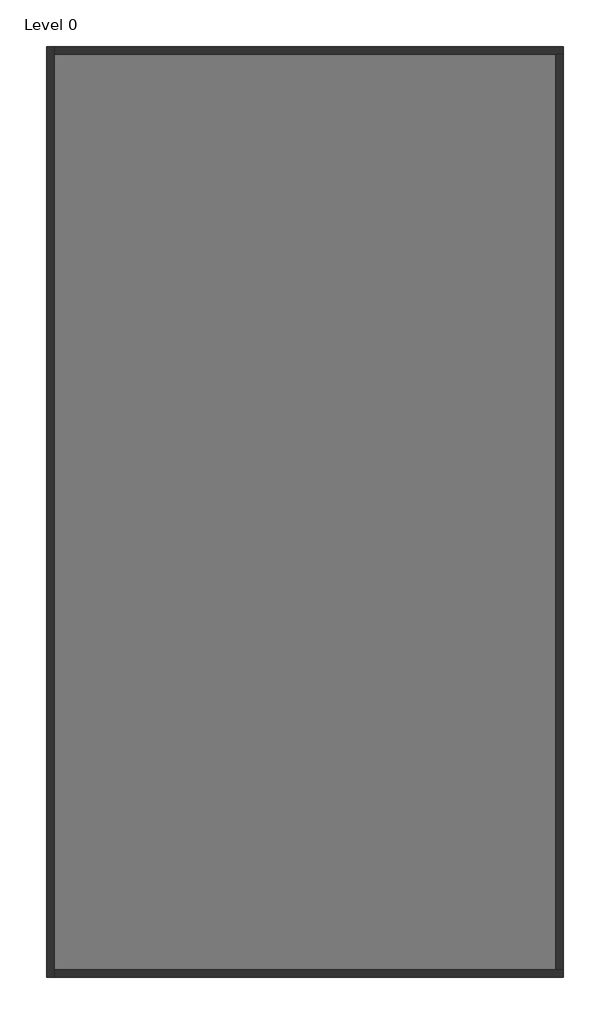
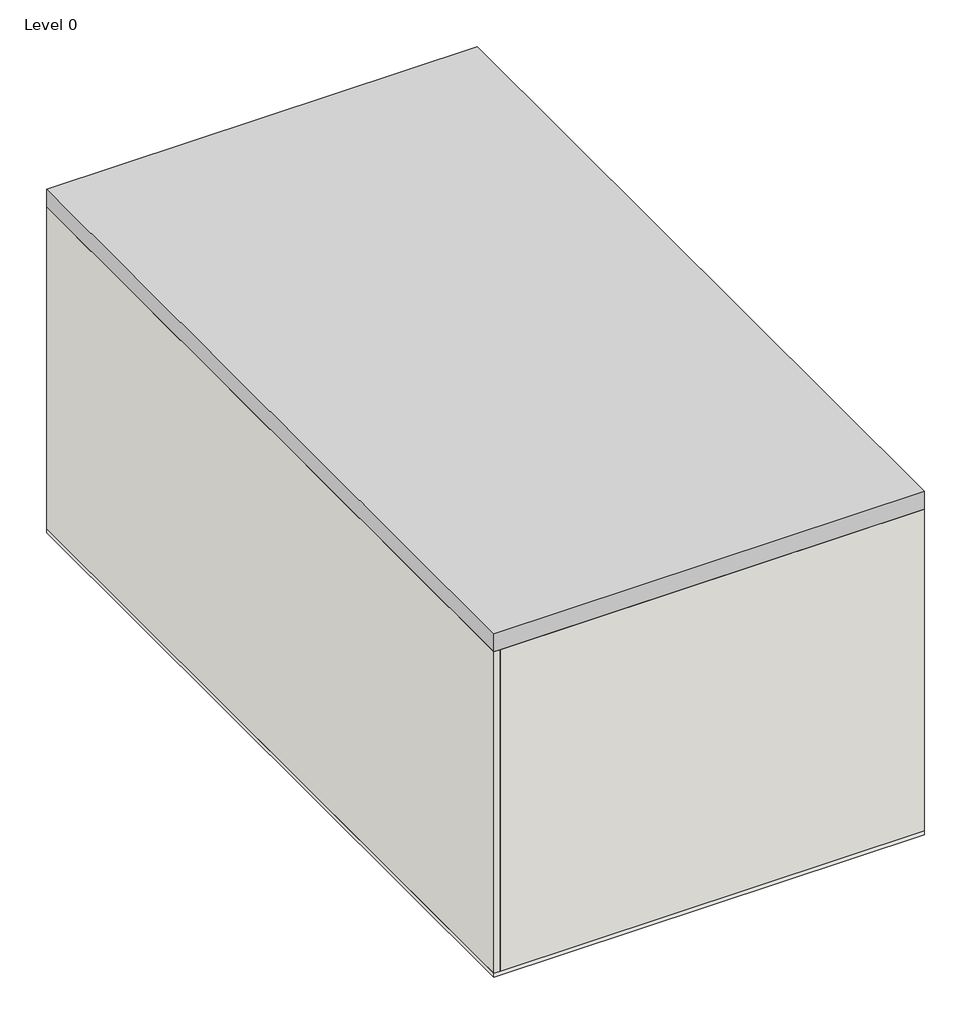
# One storey: 4 walls, 1 proxy, 1 slab.
"""IFC4 building model written with IfcOpenShell, lengths in millimetres."""

from ifc_helpers import new_model, si_unit, frame, origin, origin_with_axes, place, context, project, spatial, polyline, outline, extrude, faceted_brep, element, save

model = new_model("IFC4")

# Units and contexts
model_context = context("Model", 3, world=origin())
ifc_project = project(units=[si_unit("LENGTHUNIT", "METRE", prefix="MILLI")], contexts=[model_context])

# Site, building, storey
site = spatial("IfcSite", under=ifc_project)
building = spatial("IfcBuilding", under=site)
storey = spatial("IfcBuildingStorey", under=building, Name="Level 0", Elevation=100.0)

# Proxy
placement = place(None, origin())
element("IfcBuildingElementProxy", 1, Name="LowUrbanDensityBuilding : LowUrbanDensityBuilding", ObjectType="LowUrbanDensityBuilding : LowUrbanDensityBuilding", at=placement, inside=storey, context=model_context, shape_type="SweptSolid", body=[
    extrude(outline(polyline([(7325.2659446, 3676.2074539), (7325.2659446, -14323.7925461), (-2674.7340554, -14323.7925461), (-2674.7340554, 3676.2074539), (7325.2659446, 3676.2074539)])), origin_with_axes(), (0.0, 0.0, 1.0), 8445.0),
])

# Slab
element("IfcSlab", 2, ObjectType="Floor-Concrete_100Con", at=placement, inside=storey, context=model_context, shape_type="SweptSolid", body=[
    extrude(outline(polyline([(7325.2659446, 3676.2074539), (7325.2659446, -14323.7925461), (-2674.7340554, -14323.7925461), (-2674.7340554, 3676.2074539), (7325.2659446, 3676.2074539)])), origin_with_axes(), (0.0, 0.0, 1.0), 100.0),
])

# Walls
element("IfcWall", 3, ObjectType="Wall-Ext_25Rdr-100Blk-19P", at=placement, inside=storey, context=model_context, shape_type="Brep", body=[
    faceted_brep([(-2674.7340554, 3676.2074539, 100.0), (-2674.7340554, -14323.7925461, 100.0), (-2674.7340554, -14323.7925461, 8000.0), (-2674.7340554, 3676.2074539, 8000.0), (-2530.4340554, 3676.2074539, 100.0), (-2530.4340554, 3676.2074539, 8000.0), (-2530.4340554, 3531.9074539, 8000.0), (-2530.4340554, -14179.4925461, 8000.0), (-2530.4340554, -14323.7925461, 8000.0), (-2530.4340554, -14323.7925461, 100.0), (-2530.4340554, -14179.4925461, 100.0), (-2530.4340554, 3531.9074539, 100.0)], [[[0, 1, 2, 3]], [[4, 5, 6, 7, 8, 9, 10, 11]], [[1, 0, 4, 11, 10, 9]], [[3, 2, 8, 7, 6, 5]], [[2, 1, 9, 8]], [[0, 3, 5, 4]]]),
])
element("IfcWall", 4, ObjectType="Wall-Ext_25Rdr-100Blk-19P", at=placement, inside=storey, context=model_context, shape_type="Brep", body=[
    faceted_brep([(-2530.4340554, -14323.7925461, 100.0), (7325.2659446, -14323.7925461, 100.0), (7325.2659446, -14323.7925461, 8000.0), (-2530.4340554, -14323.7925461, 8000.0), (-2530.4340554, -14179.4925461, 100.0), (-2530.4340554, -14179.4925461, 8000.0), (7180.9659446, -14179.4925461, 8000.0), (7325.2659446, -14179.4925461, 8000.0), (7325.2659446, -14179.4925461, 100.0), (7180.9659446, -14179.4925461, 100.0)], [[[0, 1, 2, 3]], [[4, 5, 6, 7, 8, 9]], [[1, 0, 4, 9, 8]], [[3, 2, 7, 6, 5]], [[0, 3, 5, 4]], [[2, 1, 8, 7]]]),
])
element("IfcWall", 5, ObjectType="Wall-Ext_25Rdr-100Blk-19P", at=placement, inside=storey, context=model_context, shape_type="Brep", body=[
    faceted_brep([(7325.2659446, 3676.2074539, 100.0), (-2530.4340554, 3676.2074539, 100.0), (-2530.4340554, 3676.2074539, 8000.0), (7325.2659446, 3676.2074539, 8000.0), (7325.2659446, 3531.9074539, 100.0), (7325.2659446, 3531.9074539, 8000.0), (7180.9659446, 3531.9074539, 8000.0), (-2530.4340554, 3531.9074539, 8000.0), (-2530.4340554, 3531.9074539, 100.0), (7180.9659446, 3531.9074539, 100.0)], [[[0, 1, 2, 3]], [[4, 5, 6, 7, 8, 9]], [[1, 0, 4, 9, 8]], [[3, 2, 7, 6, 5]], [[2, 1, 8, 7]], [[0, 3, 5, 4]]]),
])
element("IfcWall", 6, ObjectType="Wall-Ext_25Rdr-100Blk-19P", at=placement, inside=storey, context=model_context, shape_type="SweptSolid", body=[
    extrude(outline(polyline([(7325.2659446, 3531.9074539), (7325.2659446, -14179.4925461), (7180.9659446, -14179.4925461), (7180.9659446, 3531.9074539), (7325.2659446, 3531.9074539)])), frame((0.0, 0.0, 100.0), z_axis=(0.0, 0.0, 1.0), x_axis=(1.0, 0.0, 0.0)), (0.0, 0.0, 1.0), 7900.0),
])

save(model, "model.ifc")

# Revit data of these elements
# Project information
#   Project Issue Date = "Issue Date"
#   Project Status = "Project Status"
#   Client Name = "Owner"
#   Project Address = "Enter address here"
#   Project Name = "Project Name"
#   Project Number = "Project Number"
# Type "Floor-Concrete_100Con"
#   Keynote = "E60/130"
#   Function = 0
#   Layers, outside or top first: 100 mm "Concrete" (function 1)
# Type "Wall-Ext_25Rdr-100Blk-19P"
#   Keynote = "F10"
#   Layers, outside or top first: 25.3 mm "Render, Beige, Smooth" (function 5); 100 mm "Concrete Masonry Units _Low Density" (function 1); 19 mm "Plaster" (function 5)
# Element 1 (IfcBuildingElementProxy, "LowUrbanDensityBuilding : LowUrbanDensityBuilding")
#   Phase Created = New Construction
#   Materials on its faces: "Default Form"
# Element 2 (IfcSlab, "Floor-Concrete_100Con")
#   Height Offset From Level = 0 mm
#   Phase Created = New Construction
#   Materials on its faces: "Concrete"
# Element 3 (IfcWall, "Wall-Ext_25Rdr-100Blk-19P")
#   Top Offset = 0 mm
#   Base Offset = 0 mm
#   wall height = 7900 mm
#   Phase Created = New Construction
#   Base Constraint = Level 0
#   Top Constraint = Level 2
#   Materials on its faces: "Render, Beige, Smooth", "Default Wall", "Plaster"
# Elements 4, 5, 6 (IfcWall, "Wall-Ext_25Rdr-100Blk-19P")
#   Top Offset = 0 mm
#   Base Offset = 0 mm
#   wall height = 7900 mm
#   Phase Created = New Construction
#   Base Constraint = Level 0
#   Top Constraint = Level 2
#   Materials on its faces: "Default Wall", "Render, Beige, Smooth", "Plaster"
# Materials
#   "Concrete": class "Concrete", colour RGB 120 120 120, transparency 0, Description = "Portland Cement Concrete", Cost = 0
#   "Render, Beige, Smooth": class "Generic", colour RGB 213 198 180, transparency 0, Description = "physical material", Cost = 0
#   "Concrete Masonry Units _Low Density": class "Masonry", colour RGB 181 181 181, transparency 0, Description = "Concrete masonry units", Cost = 0
#   "Plaster": class "Generic", colour RGB 249 249 249, transparency 0, Description = "Plaster", Cost = 0
#   "Default Form": class "Generic", colour RGB 185 189 196, transparency 0.5, Cost = 0
#   "Default Wall": class "Miscellaneous", colour RGB 128 128 128, transparency 0, Comments = "Rendering appearance not upgraded Rendering appearance not upgraded ", Cost = 0
